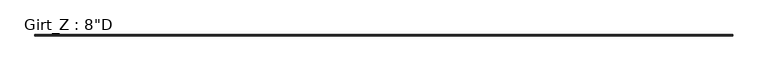
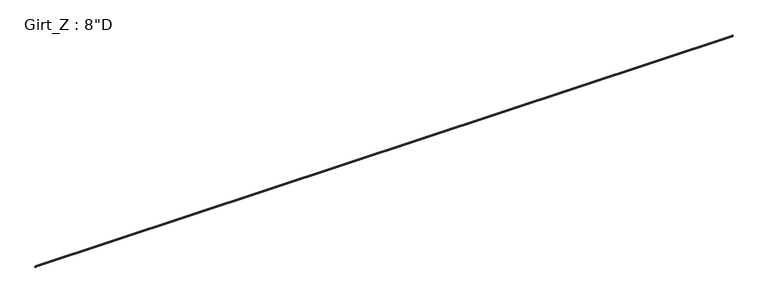
"""IFC4 building model written with IfcOpenShell, lengths in millimetres: beam geometry."""

from ifc_helpers import new_model, si_unit, point, frame, frame_2d, origin, place, context, project, spatial, polyline, circle_curve, trimmed, segment, composite_curve, outline, extrude, source, transform, mapped, element, save


def beam_24860ee2(model_context):
    return source(origin(), model_context, "Body", "SweptSolid", [
        extrude(outline(composite_curve([segment(polyline([(-63.5, 101.6), (-3.3734375, 101.6)]), True, "CONTINUOUS"), segment(trimmed(circle_curve(frame_2d((-3.3734375, 96.8375)), 4.7625), [point((-3.3734375, 101.6))], [point((1.3890625, 96.8375))], False, "CARTESIAN"), True, "CONTINUOUS"), segment(polyline([(1.3890625, 96.8375), (1.3890625, -96.8389339)]), True, "CONTINUOUS"), segment(trimmed(circle_curve(frame_2d((3.3748024, -96.8389339)), 1.9857399), [point((1.3890625, -96.8389339))], [point((3.2694106, -98.821875))], True, "CARTESIAN"), True, "CONTINUOUS"), segment(polyline([(3.2694106, -98.821875), (62.204539, -98.821875), (73.6169367, -85.221109), (75.745104, -87.0068534), (63.5, -101.6), (3.3734375, -101.6)]), True, "CONTINUOUS"), segment(trimmed(circle_curve(frame_2d((3.3734375, -96.8375)), 4.7625), [point((3.3734375, -101.6))], [point((-1.3890625, -96.8375))], False, "CARTESIAN"), True, "CONTINUOUS"), segment(polyline([(-1.3890625, -96.8375), (-1.3890625, 96.8381931)]), True, "CONTINUOUS"), segment(trimmed(circle_curve(frame_2d((-3.3741066, 96.8381931)), 1.9850441), [point((-1.3890625, 96.8381931))], [point((-3.3005807, 98.821875))], True, "CARTESIAN"), True, "CONTINUOUS"), segment(polyline([(-3.3005807, 98.821875), (-62.204539, 98.821875), (-73.6169367, 85.221109), (-75.745104, 87.0068534), (-63.5, 101.6)]), True, "CONTINUOUS")], self_intersect=False)), frame((-40485.8884766, 0.0, 0.0), z_axis=(1.0, 0.0, 0.0), x_axis=(0.0, 1.0, 0.0)), (0.0, 0.0, 1.0), 80870.1769531),
    ])


if __name__ == "__main__":
    model = new_model("IFC4")
    model_context = context("Model", 3, world=origin())
    ifc_project = project(units=[si_unit("LENGTHUNIT", "METRE", prefix="MILLI")], contexts=[model_context])
    site = spatial("IfcSite", under=ifc_project)
    building = spatial("IfcBuilding", under=site)
    placement = place(None, origin())
    beam_shape = beam_24860ee2(model_context)
    element("IfcBeam", 1, ObjectType="Girt_Z : 8\"D", at=placement, inside=building, context=model_context, shape_type="MappedRepresentation", body=[
        mapped(beam_shape, transform((0.0, 0.0, 0.0), x_axis=(1.0, 0.0, 0.0), y_axis=(0.0, 1.0, 0.0), z_axis=(0.0, 0.0, 1.0))),
    ])
    save(model, "model.ifc")

# Revit data of these elements
# Type "Girt_Z : 8\"D"
#   Web_Thickness = 0' - 0 7/64"
#   Length [instance default] = 10' - 0"
#   Leg_1 = 0' - 2 1/2"
#   Height = 0' - 8"
#   Structural Material [instance default] = none
# Element 1 (IfcBeam, "Girt_Z : 8\"D")
#   Structural Material = Steel
#   Materials on its faces: "Steel"
# Materials
#   "Steel": class "Metal", colour RGB 118 118 114, transparency 0, Description = "Steel, mill finish", Cost = 0
